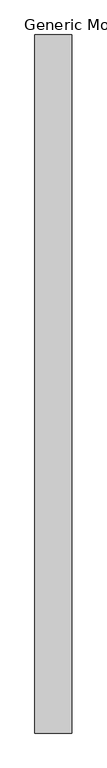
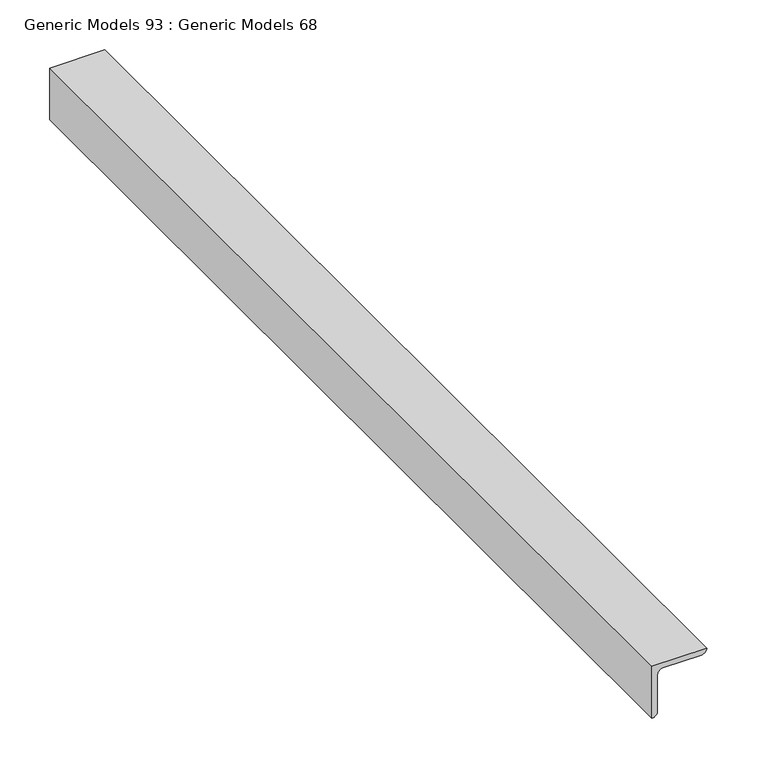
"""IFC4 building model written with IfcOpenShell, lengths in millimetres: proxy geometry, Generic Models 93 : Generic Models 68."""

from ifc_helpers import new_model, si_unit, point, frame, frame_2d, origin, place, context, project, spatial, polyline, circle_curve, trimmed, segment, composite_curve, outline, extrude, source, transform, mapped, element, save


def generic_models_93_generic_models_68_4323165a(model_context):
    return source(origin(), model_context, "Body", "SweptSolid", [
        extrude(outline(composite_curve([segment(polyline([(266004.6986952, 20536.7616945), (265941.1986952, 20536.7616945)]), True, "CONTINUOUS"), segment(trimmed(circle_curve(frame_2d((265947.5486952, 20536.7616945)), 6.35), [point((265941.1986952, 20536.7616945))], [point((265947.5486952, 20543.1116945))], False, "CARTESIAN"), True, "CONTINUOUS"), segment(polyline([(265947.5486952, 20543.1116945), (265991.9986952, 20543.1116945)]), True, "CONTINUOUS"), segment(trimmed(circle_curve(frame_2d((265991.9986952, 20549.4616945)), 6.35), [point((265991.9986952, 20543.1116945))], [point((265998.3486952, 20549.4616945))], True, "CARTESIAN"), True, "CONTINUOUS"), segment(polyline([(265998.3486952, 20549.4616945), (265998.3486952, 20593.9116945)]), True, "CONTINUOUS"), segment(trimmed(circle_curve(frame_2d((266004.6986952, 20593.9116945)), 6.35), [point((265998.3486952, 20593.9116945))], [point((266004.6986952, 20600.2616945))], False, "CARTESIAN"), True, "CONTINUOUS"), segment(polyline([(266004.6986952, 20600.2616945), (266004.6986952, 20536.7616945)]), True, "CONTINUOUS")], self_intersect=False)), frame((0.0, 18502.3764581, 0.0), z_axis=(0.0, 1.0, 0.0), x_axis=(0.0, 0.0, 1.0)), (0.0, 0.0, 1.0), 1206.5),
    ])


if __name__ == "__main__":
    model = new_model("IFC4")
    model_context = context("Model", 3, world=origin())
    ifc_project = project(units=[si_unit("LENGTHUNIT", "METRE", prefix="MILLI")], contexts=[model_context])
    site = spatial("IfcSite", under=ifc_project)
    building = spatial("IfcBuilding", under=site)
    placement = place(None, origin())
    generic_models_93_generic_models_68_shape = generic_models_93_generic_models_68_4323165a(model_context)
    element("IfcBuildingElementProxy", 1, Name="Generic Models 93 : Generic Models 68", ObjectType="Generic Models 93 : Generic Models 68", at=placement, inside=building, context=model_context, shape_type="MappedRepresentation", body=[
        mapped(generic_models_93_generic_models_68_shape, transform((0.0, 0.0, 0.0), x_axis=(1.0, 0.0, 0.0), y_axis=(0.0, 1.0, 0.0), z_axis=(0.0, 0.0, 1.0))),
    ])
    save(model, "model.ifc")

# Revit data of these elements
# Element 1 (IfcBuildingElementProxy, "Generic Models 93 : Generic Models 68")
#   Materials on its faces: "CAR DOOR RAIL: GALV. ANGLE L2 1/2 X 2 1/2 X 1/4\" @ 32\" ABOVE GRADE (PARALLEL TO HORTZ. WOOD TRIM)"
# Materials
#   "CAR DOOR RAIL: GALV. ANGLE L2 1/2 X 2 1/2 X 1/4\" @ 32\" ABOVE GRADE (PARALLEL TO HORTZ. WOOD TRIM)": class "Unassigned", colour RGB 211 211 211, transparency 0, Cost = 0
